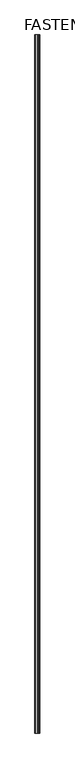
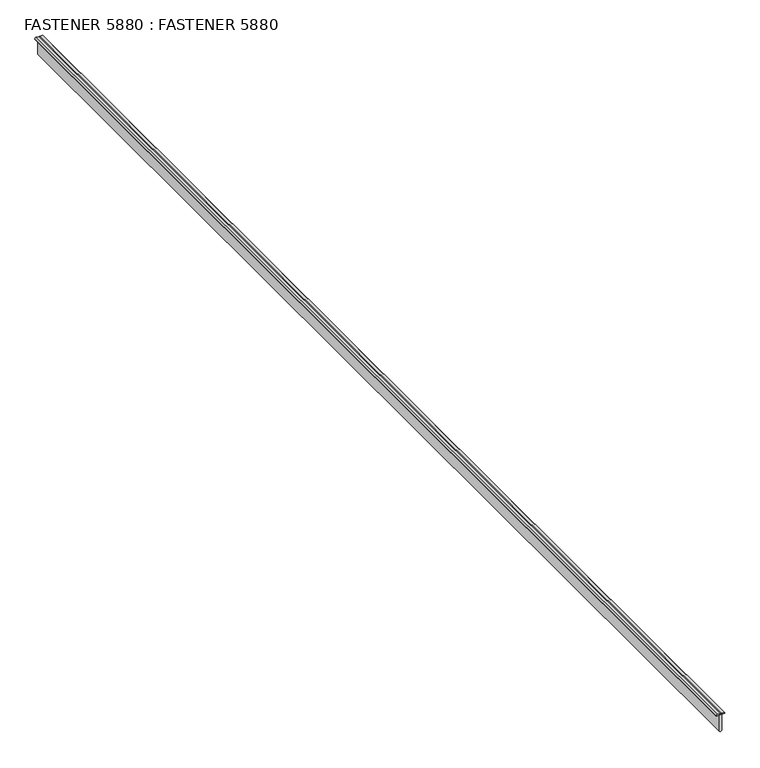
"""IFC4 building model written with IfcOpenShell, lengths in millimetres: proxy geometry, FASTENER 5880 : FASTENER 5880."""

from ifc_helpers import new_model, si_unit, frame, origin, place, context, project, spatial, polyline, outline, extrude, source, transform, mapped, element, save


def fastener_5880_fastener_5880_40db04d7(model_context):
    return source(origin(), model_context, "Body", "SweptSolid", [
        extrude(outline(polyline([(42551.3049701, 5981.517626), (42579.6987049, 5981.517626), (42579.6987049, 5977.3107075), (42550.7399648, 5977.3107075), (42549.1244121, 5978.9677221), (42551.3049701, 5981.517626)])), frame((0.0, -1052.8906574, 0.0), z_axis=(0.0, 1.0, 0.0), x_axis=(0.0, 0.0, 1.0)), (0.0, 0.0, 1.0), 1999.85),
        extrude(outline(polyline([(42580.5349921, 5972.2779845), (42579.6987049, 5972.2671879), (42579.6987049, 5986.5634932), (42580.508527, 5986.5634932), (42582.1023984, 5985.3247911), (42582.1023984, 5980.4457092), (42580.1167322, 5980.0391089), (42580.1167322, 5978.792004), (42581.7222633, 5978.792004), (42582.1288635, 5973.5166866), (42580.5349921, 5972.2779845)])), frame((0.0, -1052.8906574, 0.0), z_axis=(0.0, 1.0, 0.0), x_axis=(0.0, 0.0, 1.0)), (0.0, 0.0, 1.0), 1999.85),
    ])


if __name__ == "__main__":
    model = new_model("IFC4")
    model_context = context("Model", 3, world=origin())
    ifc_project = project(units=[si_unit("LENGTHUNIT", "METRE", prefix="MILLI")], contexts=[model_context])
    site = spatial("IfcSite", under=ifc_project)
    building = spatial("IfcBuilding", under=site)
    placement = place(None, origin())
    fastener_5880_fastener_5880_shape = fastener_5880_fastener_5880_40db04d7(model_context)
    element("IfcBuildingElementProxy", 1, Name="FASTENER 5880 : FASTENER 5880", ObjectType="FASTENER 5880 : FASTENER 5880", at=placement, inside=building, context=model_context, shape_type="MappedRepresentation", body=[
        mapped(fastener_5880_fastener_5880_shape, transform((0.0, 0.0, 0.0), x_axis=(1.0, 0.0, 0.0), y_axis=(0.0, 1.0, 0.0), z_axis=(0.0, 0.0, 1.0))),
    ])
    save(model, "model.ifc")

# Revit data of these elements
# Type "FASTENER 5880 : FASTENER 5880"
#   NameOverride = "FASTENER"
# Element 1 (IfcBuildingElementProxy, "FASTENER 5880 : FASTENER 5880")
#   Materials on its faces: "ENGINEERED PANCAKE HEAD FASTENER (NOT BY AEP-SPAN) @ 12\" O.C."
# Materials
#   "ENGINEERED PANCAKE HEAD FASTENER (NOT BY AEP-SPAN) @ 12\" O.C.": class "Unassigned", colour RGB 255 255 255, transparency 0
